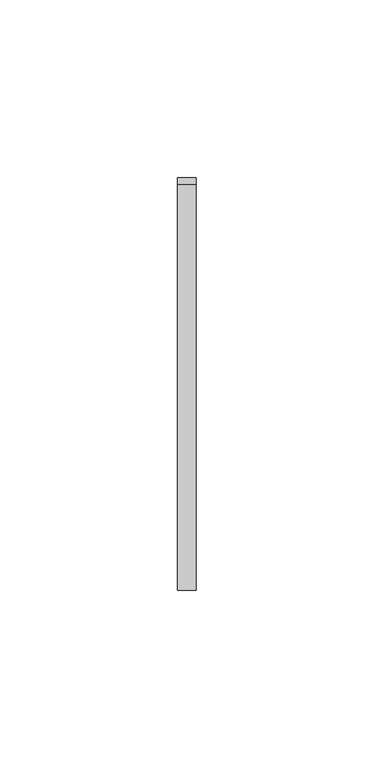
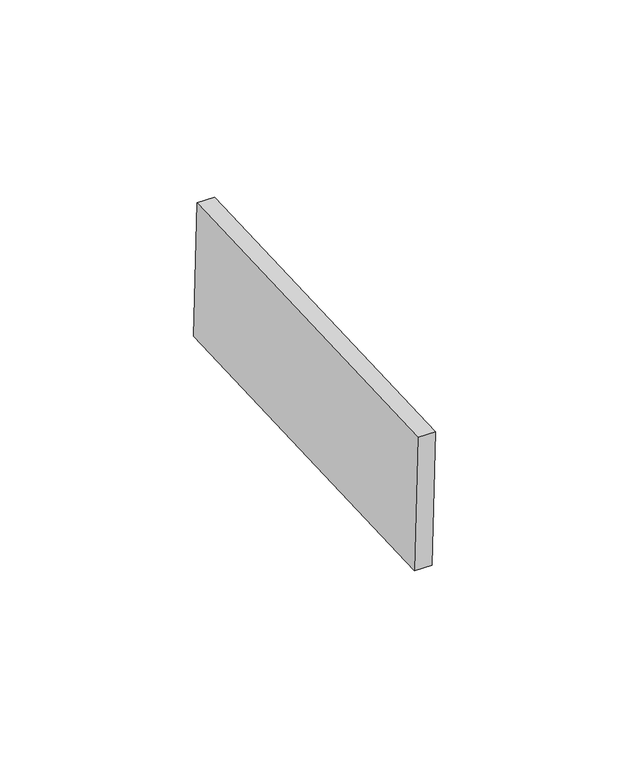
"""IFC4 building model written with IfcOpenShell, lengths in millimetres: proxy geometry, Inner panel:Inner panel:1:Inner panel:1 : Inner panel:Inner panel:300324:2:Inner panel:1:Inner panel:1 : Inner panel:Inner panel:300324:2 : Inner panel:Inner panel:1:Inner panel:1 : Inner panel:Inner panel:300324:300043:76 : Inner panel:Inner panel:1:Inner panel:1 : Inner panel:Inner panel:300324:2:Inner panel:1:Inner panel:1 : Inner panel:Inner panel:300324:2 : Inner panel:Inner panel:1:Inner panel:1 : Inner panel:Inner panel:300324:300043:308120."""

from ifc_helpers import new_model, si_unit, frame, origin, place, context, project, spatial, polyline, outline, extrude, source, transform, mapped, element, save


def generic_models_61112036(model_context):
    return source(origin(), model_context, "Body", "SweptSolid", [
        extrude(outline(polyline([(0.0, -114.3), (0.0, 0.0), (5.2138089, 0.0), (5.2138089, -114.3), (0.0, -114.3)])), frame((593123.795117, -578297.797364, 3981.6641254), z_axis=(0.0, -0.04163054471216399, 0.9991330730923527), x_axis=(-1.0, 0.0, 0.0)), (0.0, 0.0, 1.0), 43.2233908),
    ])


if __name__ == "__main__":
    model = new_model("IFC4")
    model_context = context("Model", 3, world=origin())
    ifc_project = project(units=[si_unit("LENGTHUNIT", "METRE", prefix="MILLI")], contexts=[model_context])
    site = spatial("IfcSite", under=ifc_project)
    building = spatial("IfcBuilding", under=site)
    placement = place(None, origin())
    generic_models_shape = generic_models_61112036(model_context)
    element("IfcBuildingElementProxy", 1, Name="Inner panel:Inner panel:1:Inner panel:1 : Inner panel:Inner panel:300324:2:Inner panel:1:Inner panel:1 : Inner panel:Inner panel:300324:2 : Inner panel:Inner panel:1:Inner panel:1 : Inner panel:Inner panel:300324:300043:76 : Inner panel:Inner panel:1:Inner panel:1 : Inner panel:Inner panel:300324:2:Inner panel:1:Inner panel:1 : Inner panel:Inner panel:300324:2 : Inner panel:Inner panel:1:Inner panel:1 : Inner panel:Inner panel:300324:300043:308120", ObjectType="Inner panel:Inner panel:1:Inner panel:1 : Inner panel:Inner panel:300324:2:Inner panel:1:Inner panel:1 : Inner panel:Inner panel:300324:2 : Inner panel:Inner panel:1:Inner panel:1 : Inner panel:Inner panel:300324:300043:76 : Inner panel:Inner panel:1:Inner panel:1 : Inner panel:Inner panel:300324:2:Inner panel:1:Inner panel:1 : Inner panel:Inner panel:300324:2 : Inner panel:Inner panel:1:Inner panel:1 : Inner panel:Inner panel:300324:300043:308120", at=placement, inside=building, context=model_context, shape_type="MappedRepresentation", body=[
        mapped(generic_models_shape, transform((0.0, 0.0, 0.0), x_axis=(1.0, 0.0, 0.0), y_axis=(0.0, 1.0, 0.0), z_axis=(0.0, 0.0, 1.0))),
    ])
    save(model, "model.ifc")

# Revit data of these elements
# Type "Inner panel:Inner panel:1:Inner panel:1 : Inner panel:Inner panel:300324:2:Inner panel:1:Inner panel:1 : Inner panel:Inner panel:300324:2 : Inner panel:Inner panel:1:Inner panel:1 : Inner panel:Inner panel:300324:300043:76 : Inner panel:Inner panel:1:Inner panel:1 : Inner panel:Inner panel:300324:2:Inner panel:1:Inner panel:1 : Inner panel:Inner panel:300324:2 : Inner panel:Inner panel:1:Inner panel:1 : Inner panel:Inner panel:300324:300043:308120"
#   NameOverride = "Inner panel:Inner panel:1:Inner panel:1 : Inner panel:Inner panel:300324:2:Inner panel:1:Inner panel:1 : Inner panel:Inner panel:300324:2 : Inner panel:Inner panel:1:Inner panel:1 : Inner panel:Inner panel:300324:300043:308120"
#   ObjectTypeOverride = "Inner panel:1:Inner panel:1 : Inner panel:Inner panel:300324:2 : Inner panel:Inner panel:1:Inner panel:1 : Inner panel:Inner panel:300324:300043"
#   Reference = "Inner panel"
#   Tag = "308120"
# Element 1 (IfcBuildingElementProxy, "Inner panel:Inner panel:1:Inner panel:1 : Inner panel:Inner panel:300324:2:Inner panel:1:Inner panel:1 : Inner panel:Inner panel:300324:2 : Inner panel:Inner panel:1:Inner panel:1 : Inner panel:Inner panel:300324:300043:76 : Inner panel:Inner panel:1:Inner panel:1 : Inner panel:Inner panel:300324:2:Inner panel:1:Inner panel:1 : Inner panel:Inner panel:300324:2 : Inner panel:Inner panel:1:Inner panel:1 : Inner panel:Inner panel:300324:300043:308120")
#   Materials on its faces: "SLIDING CLIP"
# Materials
#   "SLIDING CLIP": class "Generic", colour RGB 120 120 120, transparency 0, Cost = 0
